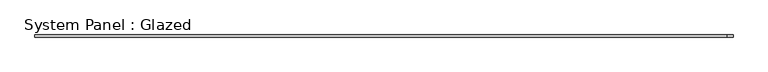
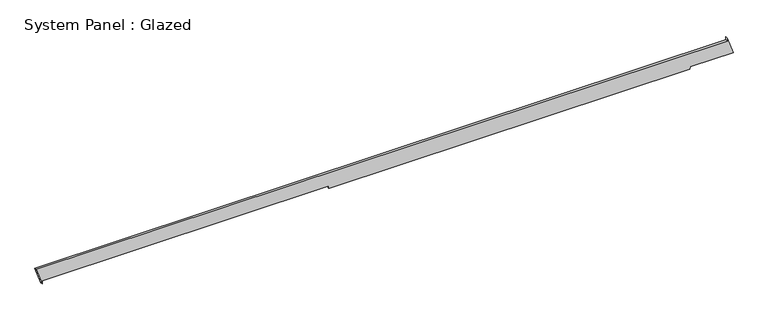
"""IFC4 building model written with IfcOpenShell, lengths in millimetres: plate geometry, System Panel : Glazed."""

from ifc_helpers import new_model, si_unit, frame, origin, place, context, project, spatial, polyline, outline, extrude, source, transform, mapped, element, save


def system_panel_glazed_dea92f41(model_context):
    return source(origin(), model_context, "Body", "SweptSolid", [
        extrude(outline(polyline([(0.0, -3959.18938), (35.3553391, -3959.18938), (35.3553391, -644.8234216), (6.9051919, -644.3080508), (6.9058184, 3528.3237203), (35.3553391, 3530.9347574), (35.3553391, 4028.1350908), (235.6861704, 3959.2885915), (200.3308313, 3959.2887727), (200.2899, -4028.1350908), (0.0, -3959.18938)])), frame((0.0, -49.5, 0.0), z_axis=(0.0, 1.0, 0.0), x_axis=(0.0, 0.0, 1.0)), (0.0, 0.0, 1.0), 25.0),
    ])


if __name__ == "__main__":
    model = new_model("IFC4")
    model_context = context("Model", 3, world=origin())
    ifc_project = project(units=[si_unit("LENGTHUNIT", "METRE", prefix="MILLI")], contexts=[model_context])
    site = spatial("IfcSite", under=ifc_project)
    building = spatial("IfcBuilding", under=site)
    placement = place(None, origin())
    system_panel_glazed_shape = system_panel_glazed_dea92f41(model_context)
    element("IfcPlate", 1, ObjectType="System Panel : Glazed", at=placement, inside=building, context=model_context, shape_type="MappedRepresentation", body=[
        mapped(system_panel_glazed_shape, transform((0.0, 0.0, 0.0), x_axis=(1.0, 0.0, 0.0), y_axis=(0.0, 1.0, 0.0), z_axis=(0.0, 0.0, 1.0))),
    ])
    save(model, "model.ifc")

# Revit data of these elements
# Element 1 (IfcPlate, "System Panel : Glazed")
#   Materials on its faces: "Glass"
# Materials
#   "Glass": class "Glass", colour RGB 218 227 224, transparency 0.85, Description = "Soda Lime Glass", Cost = 0
